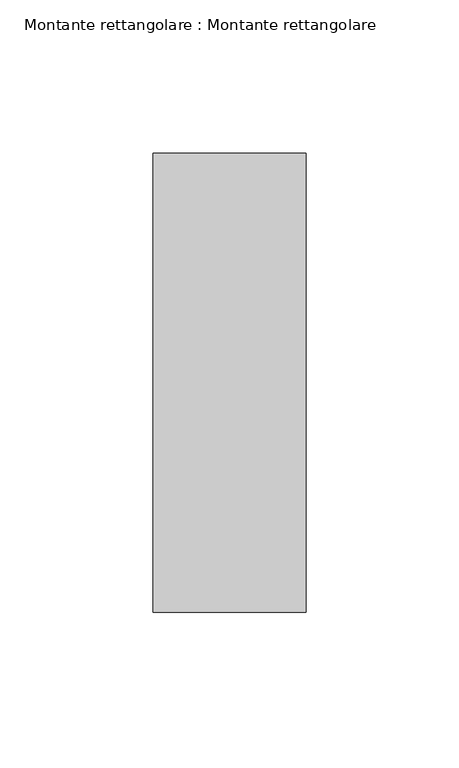
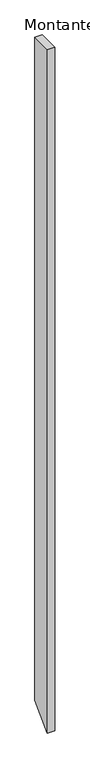
"""IFC4 building model written with IfcOpenShell, lengths in millimetres: member geometry, Montante rettangolare : Montante rettangolare."""

from ifc_helpers import new_model, si_unit, frame, origin, place, context, project, spatial, polyline, outline, extrude, source, transform, mapped, element, save


def montante_rettangolare_montante_rettangolare_370ce85d(model_context):
    return source(origin(), model_context, "Body", "SweptSolid", [
        extrude(outline(polyline([(-75.0, 0.0), (75.0, 0.0), (75.0, -4845.0), (-75.0, -4995.0), (-75.0, 0.0)])), frame((-50.0, 0.0, 0.0), z_axis=(1.0, 0.0, 0.0), x_axis=(0.0, 1.0, 0.0)), (0.0, 0.0, 1.0), 50.0),
    ])


if __name__ == "__main__":
    model = new_model("IFC4")
    model_context = context("Model", 3, world=origin())
    ifc_project = project(units=[si_unit("LENGTHUNIT", "METRE", prefix="MILLI")], contexts=[model_context])
    site = spatial("IfcSite", under=ifc_project)
    building = spatial("IfcBuilding", under=site)
    placement = place(None, origin())
    montante_rettangolare_montante_rettangolare_shape = montante_rettangolare_montante_rettangolare_370ce85d(model_context)
    element("IfcMember", 1, ObjectType="Montante rettangolare : Montante rettangolare", at=placement, inside=building, context=model_context, shape_type="MappedRepresentation", body=[
        mapped(montante_rettangolare_montante_rettangolare_shape, transform((0.0, 0.0, 0.0), x_axis=(1.0, 0.0, 0.0), y_axis=(0.0, 1.0, 0.0), z_axis=(0.0, 0.0, 1.0))),
    ])
    save(model, "model.ifc")

# Revit data of these elements
# Type "Montante rettangolare : Montante rettangolare"
#   built-in parameter 1007304 = 0.492126 (stored number, unit not read)
#   built-in parameter 1007301 = 0.082021 (stored number, unit not read)
#   built-in parameter 1007300 = 0.082021 (stored number, unit not read)
# Element 1 (IfcMember, "Montante rettangolare : Montante rettangolare")
#   Materials on its faces: "Acciaio"
# Materials
#   "Acciaio": class "Metallo", colour RGB 247 247 247, transparency 0, Description = "Acciaio, finitura zigrinata", Cost = 0
